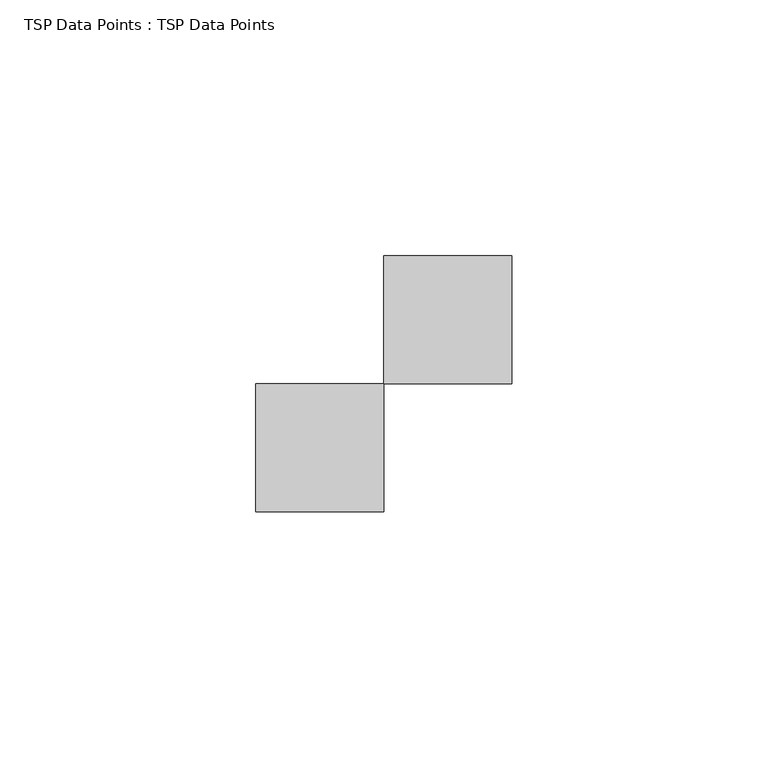
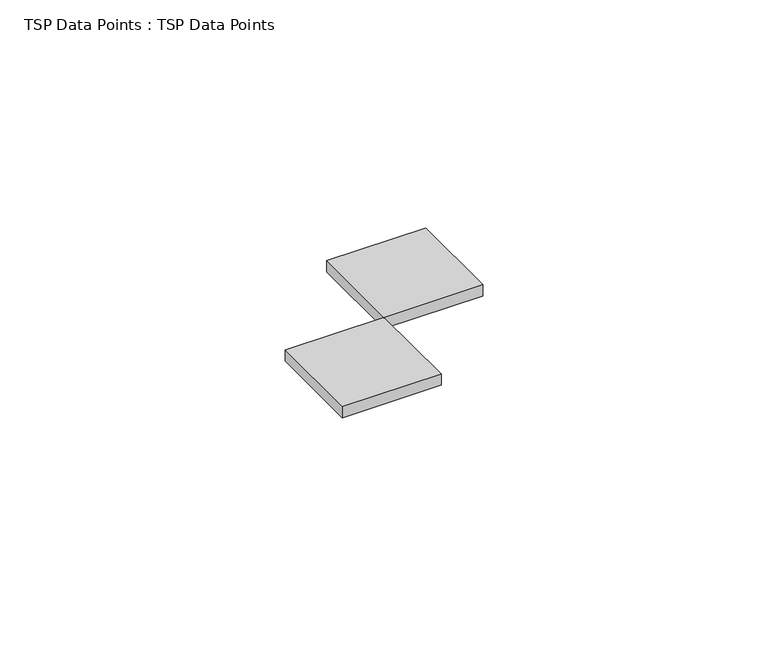
"""IFC4 building model written with IfcOpenShell, lengths in millimetres: proxy geometry, TSP Data Points : TSP Data Points."""

from ifc_helpers import new_model, si_unit, origin, origin_with_axes, place, context, project, spatial, polyline, outline, extrude, source, transform, mapped, element, save


def tsp_data_points_tsp_data_points_4d1be355(model_context):
    return source(origin(), model_context, "Body", "SweptSolid", [
        extrude(outline(polyline([(-25.0, 0.0), (-25.0, 25.0), (0.0, 25.0), (0.0, 0.0), (-25.0, 0.0)])), origin_with_axes(), (0.0, 0.0, 1.0), 3.0),
        extrude(outline(polyline([(-50.0, 0.0), (-25.0, 0.0), (-25.0, -25.0), (-50.0, -25.0), (-50.0, 0.0)])), origin_with_axes(), (0.0, 0.0, 1.0), 3.0),
    ])


if __name__ == "__main__":
    model = new_model("IFC4")
    model_context = context("Model", 3, world=origin())
    ifc_project = project(units=[si_unit("LENGTHUNIT", "METRE", prefix="MILLI")], contexts=[model_context])
    site = spatial("IfcSite", under=ifc_project)
    building = spatial("IfcBuilding", under=site)
    placement = place(None, origin())
    tsp_data_points_tsp_data_points_shape = tsp_data_points_tsp_data_points_4d1be355(model_context)
    element("IfcBuildingElementProxy", 1, Name="TSP Data Points : TSP Data Points", ObjectType="TSP Data Points : TSP Data Points", at=placement, inside=building, context=model_context, shape_type="MappedRepresentation", body=[
        mapped(tsp_data_points_tsp_data_points_shape, transform((0.0, 0.0, 0.0), x_axis=(1.0, 0.0, 0.0), y_axis=(0.0, 1.0, 0.0), z_axis=(0.0, 0.0, 1.0))),
    ])
    save(model, "model.ifc")

# Revit data of these elements
# Type "TSP Data Points : TSP Data Points"
#   Model = "TSP_ELECDATP"
#   Default Elevation = 0
# Element 1 (IfcBuildingElementProxy, "TSP Data Points : TSP Data Points")
#   Materials on its faces: "Aluminum, Anodized Red", "Plastic, Opaque Black"
# Materials
#   "Aluminum, Anodized Red": class "Metal", colour RGB 120 120 120, transparency 0, Description = "Anodized aluminum, red", Cost = 0
#   "Plastic, Opaque Black": class "Plastic", colour RGB 0 0 0, transparency 0.7, Description = "Plastic, generic, opaque black", Cost = 0
